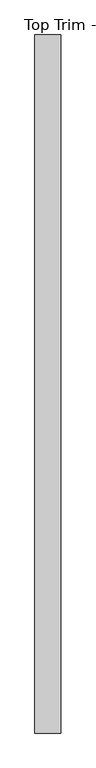
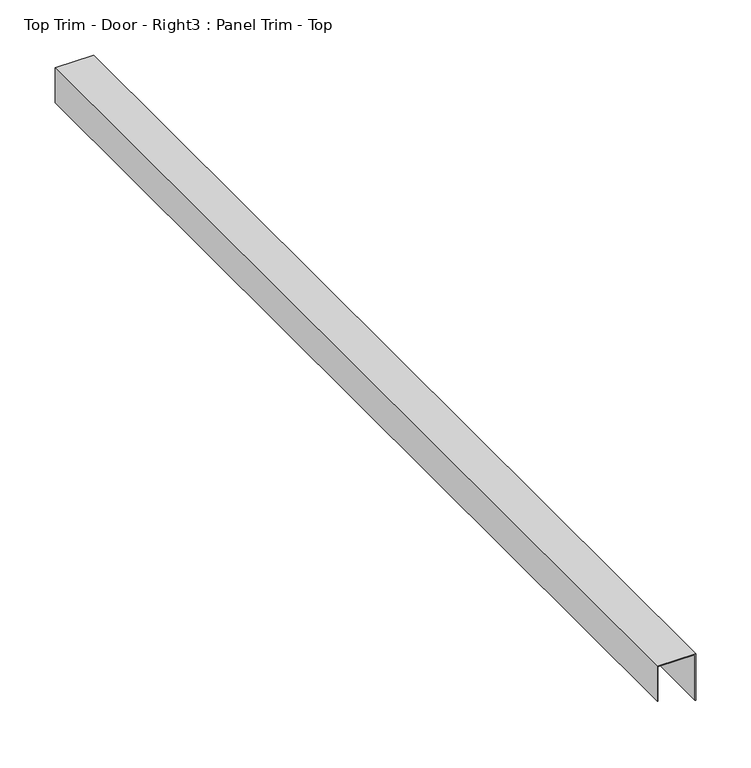
"""IFC4 building model written with IfcOpenShell, lengths in millimetres: proxy geometry, Top Trim - Door - Right3 : Panel Trim - Top."""

from ifc_helpers import new_model, si_unit, frame, origin, place, context, project, spatial, polyline, outline, extrude, source, transform, mapped, element, save


def top_trim_door_right3_panel_trim_top_e01be231(model_context):
    return source(origin(), model_context, "Body", "SweptSolid", [
        extrude(outline(polyline([(2438.4, 587327.0060739), (2438.4, 587365.8934739), (2387.6, 587365.8934739), (2387.6, 587366.6808739), (2439.19375, 587366.6808739), (2439.19375, 587326.2186739), (2400.3, 587326.2186739), (2400.3, 587327.0060739), (2438.4, 587327.0060739)])), frame((0.0, -536301.7038841, 0.0), z_axis=(0.0, 1.0, 0.0), x_axis=(0.0, 0.0, 1.0)), (0.0, 0.0, 1.0), 1093.7875),
    ])


if __name__ == "__main__":
    model = new_model("IFC4")
    model_context = context("Model", 3, world=origin())
    ifc_project = project(units=[si_unit("LENGTHUNIT", "METRE", prefix="MILLI")], contexts=[model_context])
    site = spatial("IfcSite", under=ifc_project)
    building = spatial("IfcBuilding", under=site)
    placement = place(None, origin())
    top_trim_door_right3_panel_trim_top_shape = top_trim_door_right3_panel_trim_top_e01be231(model_context)
    element("IfcBuildingElementProxy", 1, Name="Top Trim - Door - Right3 : Panel Trim - Top", ObjectType="Top Trim - Door - Right3 : Panel Trim - Top", at=placement, inside=building, context=model_context, shape_type="MappedRepresentation", body=[
        mapped(top_trim_door_right3_panel_trim_top_shape, transform((0.0, 0.0, 0.0), x_axis=(1.0, 0.0, 0.0), y_axis=(0.0, 1.0, 0.0), z_axis=(0.0, 0.0, 1.0))),
    ])
    save(model, "model.ifc")

# Revit data of these elements
# Element 1 (IfcBuildingElementProxy, "Top Trim - Door - Right3 : Panel Trim - Top")
#   Materials on its faces: "EDGE TRIM BY MTL PANEL MFR."
# Materials
#   "EDGE TRIM BY MTL PANEL MFR.": class "Generic", colour RGB 239 242 240, transparency 0, Cost = 0
